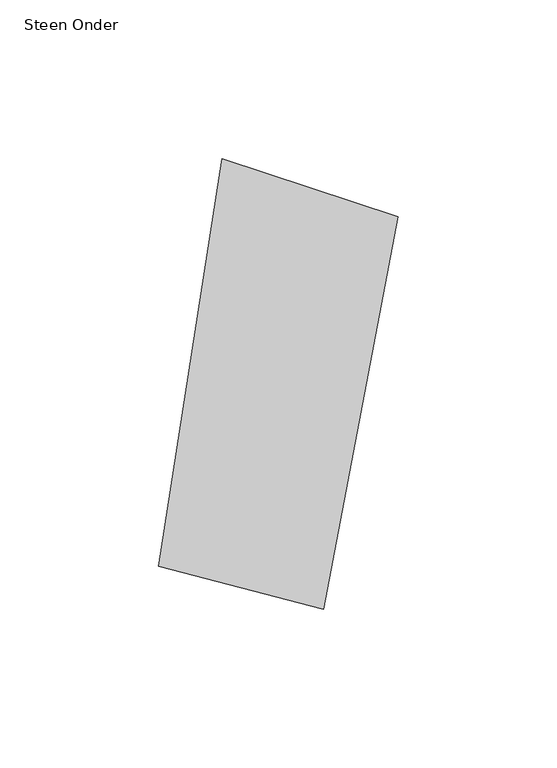
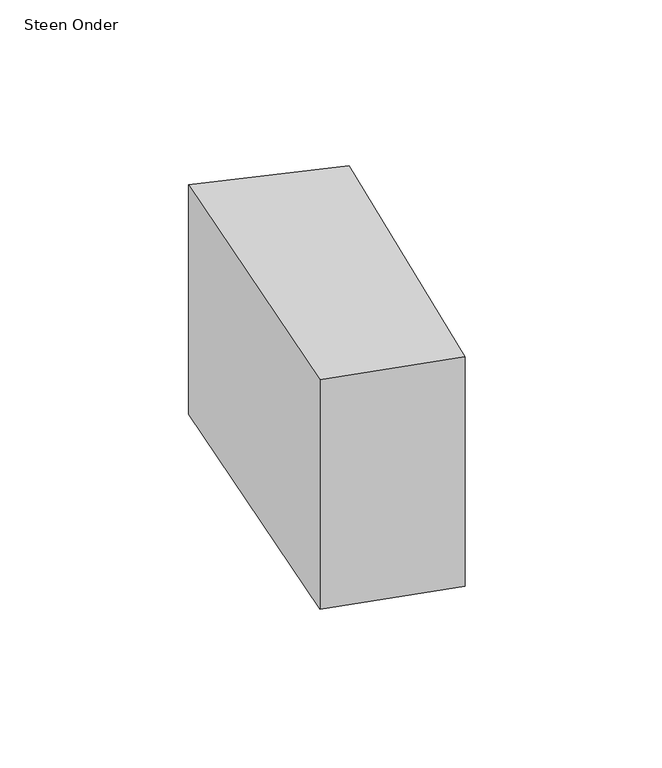
"""IFC4 building model written with IfcOpenShell, lengths in millimetres: proxy geometry, 00_GMA_steen_versie_4 : Steen Onder."""

import ifcopenshell
import ifcopenshell.guid

model = None  # the IFC model being written
_history = None  # IfcOwnerHistory: only IFC2X3 demands one
_inside = {}  # id of a spatial element -> (the spatial element, [elements in it])
_under = {}  # id of a project, library or spatial element -> (it, [spatial elements below it])
_declared = {}  # id of a project -> (the project, [libraries it declares])
_typed = {}  # id of a type object -> (the type object, [elements of that type])
_made_of = {}  # id of a material, layer set ... -> (it, [elements and type objects made of it])


def new_model(schema):
    """Start an empty IFC model of exactly this schema.

    Asked for "IFC4X3", IfcOpenShell would pick the latest addendum, in which some entities
    have other attributes; the version numbers below select the first issue.
    IFC2X3 requires an IfcOwnerHistory on every rooted entity: one is made here for all.
    """
    global model, _history
    if schema == "IFC4X3":
        model = ifcopenshell.file(schema_version=(4, 3, 0, 0))
    else:
        model = ifcopenshell.file(schema=schema)
    _inside.clear()
    _under.clear()
    _declared.clear()
    _typed.clear()
    _made_of.clear()
    _history = None
    if model.schema == "IFC2X3":
        org = make("IfcOrganization", Name="unknown")
        user = make(
            "IfcPersonAndOrganization",
            ThePerson=make("IfcPerson", FamilyName="unknown"),
            TheOrganization=org,
        )
        app = make(
            "IfcApplication",
            ApplicationDeveloper=org,
            Version="unknown",
            ApplicationFullName="unknown",
            ApplicationIdentifier="unknown",
        )
        _history = make(
            "IfcOwnerHistory",
            OwningUser=user,
            OwningApplication=app,
            ChangeAction="ADDED",
            CreationDate=0,
        )
    return model


def make(cls, **values):
    """One entity of the class cls with the attributes given. An attribute that is None is left unset."""
    return model.create_entity(
        cls, **{name: value for name, value in values.items() if value is not None}
    )


def rooted(cls, **values):
    """An entity with a GlobalId (a new one), such as an element, a storey or a relation."""
    return make(cls, GlobalId=ifcopenshell.guid.new(), OwnerHistory=_history, **values)


def si_unit(unit_type, name, prefix=None):
    """IfcSIUnit, for example si_unit("LENGTHUNIT", "METRE", prefix="MILLI")."""
    return make("IfcSIUnit", UnitType=unit_type, Prefix=prefix, Name=name)


def assignment(units):
    """IfcUnitAssignment: the units of a project."""
    return None if units is None else make("IfcUnitAssignment", Units=units)


def point(xyz):
    """IfcCartesianPoint."""
    return None if xyz is None else make("IfcCartesianPoint", Coordinates=xyz)


def direction(xyz):
    """IfcDirection."""
    return None if xyz is None else make("IfcDirection", DirectionRatios=xyz)


def frame(location, z_axis=None, x_axis=None):
    """IfcAxis2Placement3D, a coordinate frame: its origin and axes. An axis left out is left unset."""
    return make(
        "IfcAxis2Placement3D",
        Location=point(location),
        Axis=direction(z_axis),
        RefDirection=direction(x_axis),
    )


def origin():
    """The frame at (0, 0, 0) with its axes left unset."""
    return frame((0.0, 0.0, 0.0))


def origin_with_axes():
    """The frame at (0, 0, 0) with the z axis (0, 0, 1) and the x axis (1, 0, 0) written out."""
    return frame((0.0, 0.0, 0.0), z_axis=(0.0, 0.0, 1.0), x_axis=(1.0, 0.0, 0.0))


def place(relative_to, where):
    """IfcLocalPlacement: puts the frame where relative to a parent placement (None: the world)."""
    return make(
        "IfcLocalPlacement", PlacementRelTo=relative_to, RelativePlacement=where
    )


def context(
    kind, dimensions, precision=None, world=None, true_north=None, identifier=None
):
    """IfcGeometricRepresentationContext, for example the 3D "Model" context."""
    return make(
        "IfcGeometricRepresentationContext",
        ContextIdentifier=identifier,
        ContextType=kind,
        CoordinateSpaceDimension=dimensions,
        Precision=precision,
        WorldCoordinateSystem=world,
        TrueNorth=true_north,
    )


def project(units=None, contexts=None):
    """IfcProject with its units and contexts."""
    return rooted(
        "IfcProject",
        Name="project",
        RepresentationContexts=contexts,
        UnitsInContext=assignment(units),
    )


def spatial(cls, under=None, at=None, **own):
    """A site, building, storey or space (cls), placed at a placement, below another one or the project."""
    s = rooted(cls, ObjectPlacement=at, **own)
    if under is not None:
        _under.setdefault(under.id(), (under, []))[1].append(s)
    return s


def polyline(points):
    """IfcPolyline through the points."""
    return make("IfcPolyline", Points=[point(p) for p in points])


def outline(outer, holes=None, kind="AREA"):
    """IfcArbitraryClosedProfileDef: a profile drawn as a closed curve; with holes, ...WithVoids."""
    if holes is None:
        return make("IfcArbitraryClosedProfileDef", ProfileType=kind, OuterCurve=outer)
    return make(
        "IfcArbitraryProfileDefWithVoids",
        ProfileType=kind,
        OuterCurve=outer,
        InnerCurves=holes,
    )


def extrude(swept, where, along, depth):
    """IfcExtrudedAreaSolid: the profile swept, set in the frame where, extruded along a direction by depth."""
    return make(
        "IfcExtrudedAreaSolid",
        SweptArea=swept,
        Position=where,
        ExtrudedDirection=direction(along),
        Depth=depth,
    )


def shape(context_of_items, identifier, shape_type, items):
    """IfcShapeRepresentation: the items that make up one representation, for example the "Body"."""
    return make(
        "IfcShapeRepresentation",
        ContextOfItems=context_of_items,
        RepresentationIdentifier=identifier,
        RepresentationType=shape_type,
        Items=items,
    )


def source(mapping_origin, context_of_items, identifier, shape_type, items):
    """IfcRepresentationMap: a shape defined once, which mapped items show again and again."""
    return make(
        "IfcRepresentationMap",
        MappingOrigin=mapping_origin,
        MappedRepresentation=shape(context_of_items, identifier, shape_type, items),
    )


def transform(
    local_origin,
    x_axis=None,
    y_axis=None,
    z_axis=None,
    scale=None,
    scale2=None,
    scale3=None,
    uniform=True,
):
    """IfcCartesianTransformationOperator3D, or its non-uniform kind. x_axis, y_axis, z_axis: its Axis1, 2, 3."""
    if uniform:
        return make(
            "IfcCartesianTransformationOperator3D",
            Axis1=direction(x_axis),
            Axis2=direction(y_axis),
            LocalOrigin=point(local_origin),
            Scale=scale,
            Axis3=direction(z_axis),
        )
    return make(
        "IfcCartesianTransformationOperator3DnonUniform",
        Axis1=direction(x_axis),
        Axis2=direction(y_axis),
        LocalOrigin=point(local_origin),
        Scale=scale,
        Axis3=direction(z_axis),
        Scale2=scale2,
        Scale3=scale3,
    )


def mapped(mapping_source, mapping_target):
    """IfcMappedItem: shows the shape of a source again, moved by a transform."""
    return make(
        "IfcMappedItem", MappingSource=mapping_source, MappingTarget=mapping_target
    )


def made_of(thing, what):
    """Note that an element or type object is made of a material, layer set ...; save() writes the relation."""
    if what is not None:
        _made_of.setdefault(what.id(), (what, []))[1].append(thing)
    return thing


def element(
    cls,
    number,
    at=None,
    inside=None,
    cuts=None,
    type_object=None,
    material=None,
    context=None,
    identifier="Body",
    shape_type=None,
    held_by="IfcProductDefinitionShape",
    body=None,
    shapes=None,
    **own,
):
    """One element of the class cls, such as IfcWall. Its Tag is "e" and its number.

    at: its placement. inside: the storey or other place that contains it. cuts: it is an
    opening in that element (IfcRelVoidsElement). A single representation is given by context,
    identifier, shape_type and body (its items); several are given by shapes. held_by: the class
    of the entity that holds the representations. save() writes the other relations.
    """
    e = rooted(cls, Tag="e%d" % number, ObjectPlacement=at, **own)
    if body is not None:
        shapes = [shape(context, identifier, shape_type, body)]
    if shapes is not None:
        e.Representation = make(held_by, Representations=shapes)
    if inside is not None:
        _inside.setdefault(inside.id(), (inside, []))[1].append(e)
    if cuts is not None:
        rooted(
            "IfcRelVoidsElement", RelatingBuildingElement=cuts, RelatedOpeningElement=e
        )
    if type_object is not None:
        _typed.setdefault(type_object.id(), (type_object, []))[1].append(e)
    return made_of(e, material)


def aggregate(whole, parts):
    """IfcRelAggregates: a whole, such as a stair, and the parts it consists of."""
    return rooted("IfcRelAggregates", RelatingObject=whole, RelatedObjects=parts)


def save(model, path):
    """Write the relations noted so far, then the file.

    IfcRelAggregates (storeys below a building ...), IfcRelContainedInSpatialStructure (elements
    in a storey), IfcRelDefinesByType, IfcRelAssociatesMaterial and IfcRelDeclares: one each for
    every whole, place, type object, material and project.
    """
    for whole, parts in _under.values():
        aggregate(whole, parts)
    for where, things in _inside.values():
        rooted(
            "IfcRelContainedInSpatialStructure",
            RelatedElements=things,
            RelatingStructure=where,
        )
    for kind, things in _typed.values():
        rooted("IfcRelDefinesByType", RelatedObjects=things, RelatingType=kind)
    for what, things in _made_of.values():
        rooted("IfcRelAssociatesMaterial", RelatedObjects=things, RelatingMaterial=what)
    for by, libraries in _declared.values():
        rooted("IfcRelDeclares", RelatingContext=by, RelatedDefinitions=libraries)
    model.write(path)


def steen_onder_2adaac91(model_context):
    return source(origin(), model_context, "Body", "SweptSolid", [
        extrude(outline(polyline([(112.1090963, 129.5760924), (88.5653137, 5.8607567), (36.5514172, 19.3531164), (56.6450748, 147.8955626), (112.1090963, 129.5760924)])), origin_with_axes(), (0.0, 0.0, 1.0), 100.0),
    ])


if __name__ == "__main__":
    model = new_model("IFC4")
    model_context = context("Model", 3, world=origin())
    ifc_project = project(units=[si_unit("LENGTHUNIT", "METRE", prefix="MILLI")], contexts=[model_context])
    site = spatial("IfcSite", under=ifc_project)
    building = spatial("IfcBuilding", under=site)
    placement = place(None, origin())
    steen_onder_shape = steen_onder_2adaac91(model_context)
    element("IfcBuildingElementProxy", 1, Name="00_GMA_steen_versie_4 : Steen Onder", ObjectType="00_GMA_steen_versie_4 : Steen Onder", at=placement, inside=building, context=model_context, shape_type="MappedRepresentation", body=[
        mapped(steen_onder_shape, transform((0.0, 0.0, 0.0), x_axis=(1.0, 0.0, 0.0), y_axis=(0.0, 1.0, 0.0), z_axis=(0.0, 0.0, 1.0))),
    ])
    save(model, "model.ifc")

# Revit data of these elements
# Type "00_GMA_steen_versie_4 : Steen Onder"
#   StootVoegHalfBoven [instance default] = 5 mm
#   StootVoegHalf [instance default] = 5 mm
#   StootVoegBreedteOnder = 10 mm
#   StootVoegBreedteBoven = 10 mm
#   Steendikte = 100 mm
#   LintVoegOnderHalf = 0 mm
#   LintVoegOnder = 0 mm
#   LintVoegBovenHalf = 5 mm
#   LintVoegBoven = 10 mm
#   materiaal = none
#   MateriaalVoeg = none
#   Default Elevation = 0
